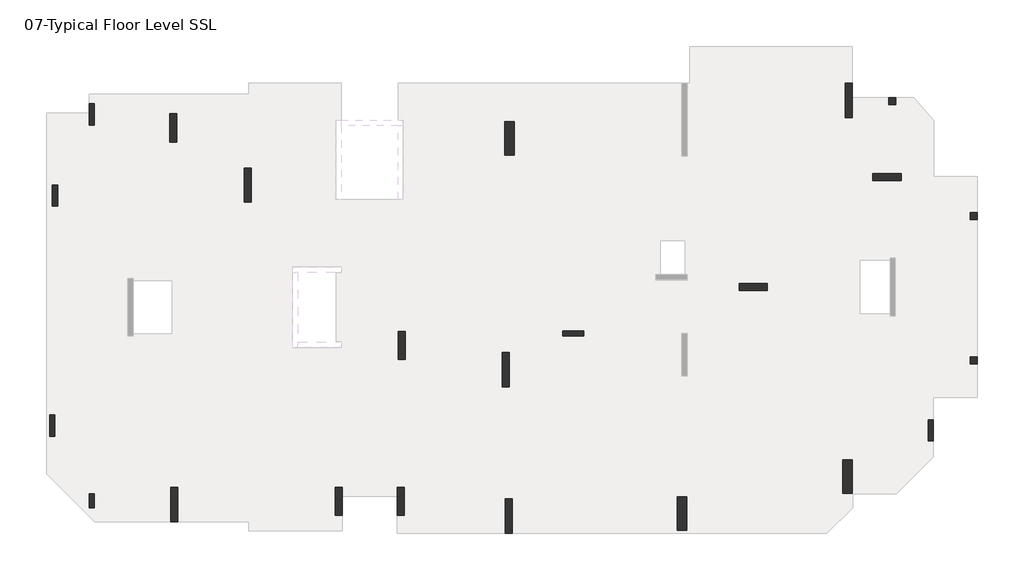
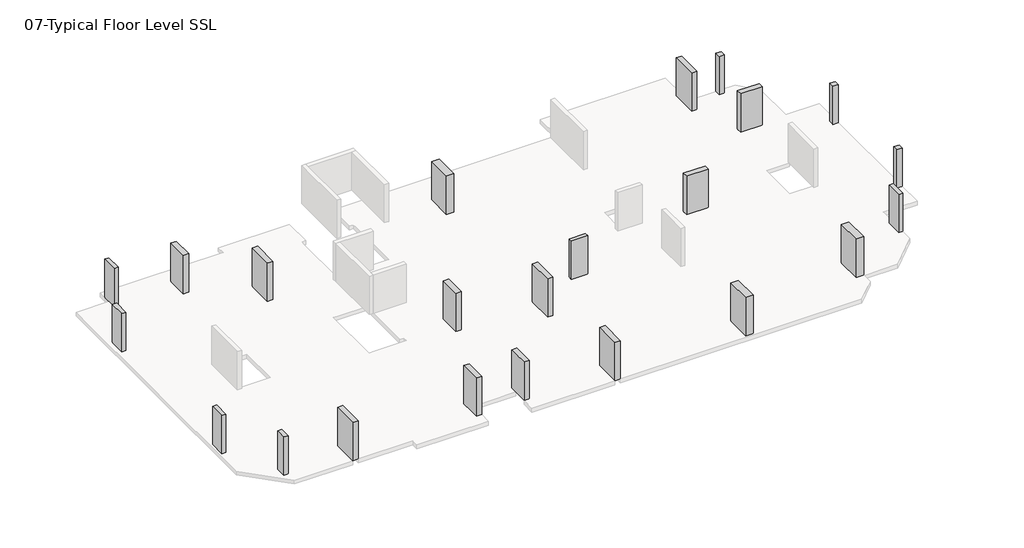
# One storey, part 2 of 2: 23 columns.
"""IFC4 building model written with IfcOpenShell, lengths in millimetres."""

from ifc_helpers import new_model, si_unit, origin, place, context, project, spatial, faceted_brep, element, save

model = new_model("IFC4")

# Units and contexts
model_context = context("Model", 3, world=origin())
ifc_project = project(units=[si_unit("LENGTHUNIT", "METRE", prefix="MILLI")], contexts=[model_context])

# Site, building, storey
site = spatial("IfcSite", under=ifc_project)
building = spatial("IfcBuilding", under=site)
storey = spatial("IfcBuildingStorey", under=building, Name="07-Typical Floor Level SSL", Elevation=15000.0)

# Columns
placement = place(None, origin())
element("IfcColumn", 1, ObjectType="M_Concrete-Rectangular-Column : C-1 (400 x 400mm)", at=placement, inside=storey, context=model_context, shape_type="Brep", body=[
    faceted_brep([(52549.9999998, 16712.0, 15000.0), (52549.9999998, 16312.0, 15000.0), (52149.9999998, 16312.0, 15000.0), (52149.9999998, 16712.0, 15000.0), (52549.9999998, 16712.0, 18000.0), (52549.9999998, 16312.0, 18000.0), (52549.9999998, 16312.0, 17700.0), (52549.9999998, 16712.0, 17700.0), (52149.9999998, 16312.0, 18000.0), (52149.9999998, 16312.0, 17700.0), (52149.9999998, 16712.0, 18000.0), (52149.9999998, 16712.0, 17700.0)], [[[0, 1, 2, 3]], [[4, 5, 6, 1, 0, 7]], [[5, 8, 9, 2, 1, 6]], [[8, 10, 11, 3, 2, 9]], [[10, 4, 7, 0, 3, 11]], [[4, 10, 8, 5]]]),
])
element("IfcColumn", 2, ObjectType="M_Concrete-Rectangular-Column : C-1 (400 x 400mm)", at=placement, inside=storey, context=model_context, shape_type="Brep", body=[
    faceted_brep([(47898.6337868, 23252.0, 15000.0), (47898.6337868, 22852.0, 15000.0), (47498.6337868, 22852.0, 15000.0), (47498.6337868, 23252.0, 15000.0), (47898.6337868, 23252.0, 18000.0), (47898.6337868, 22852.0, 18000.0), (47898.6337868, 22852.0, 17700.0), (47498.6337868, 22852.0, 18000.0), (47498.6337868, 22852.0, 17700.0), (47498.6337868, 23252.0, 18000.0)], [[[0, 1, 2, 3]], [[4, 5, 6, 1, 0]], [[5, 7, 8, 2, 1, 6]], [[7, 9, 3, 2, 8]], [[9, 4, 0, 3]], [[4, 9, 7, 5]]]),
])
element("IfcColumn", 3, ObjectType="M_Concrete-Rectangular-Column : C-1 (400 x 400mm)", at=placement, inside=storey, context=model_context, shape_type="Brep", body=[
    faceted_brep([(52549.9999998, 8504.0039609, 15000.0), (52549.9999998, 8104.0039609, 15000.0), (52149.9999998, 8104.0039609, 15000.0), (52149.9999998, 8504.0039609, 15000.0), (52549.9999998, 8504.0039609, 18000.0), (52549.9999998, 8104.0039609, 18000.0), (52549.9999998, 8104.0039609, 17700.0), (52549.9999998, 8504.0039609, 17700.0), (52149.9999998, 8104.0039609, 18000.0), (52149.9999998, 8104.0039609, 17700.0), (52149.9999998, 8504.0039609, 18000.0), (52149.9999998, 8504.0039609, 17700.0)], [[[0, 1, 2, 3]], [[4, 5, 6, 1, 0, 7]], [[5, 8, 9, 2, 1, 6]], [[8, 10, 11, 3, 2, 9]], [[10, 4, 7, 0, 3, 11]], [[4, 10, 8, 5]]]),
])
element("IfcColumn", 4, ObjectType="M_Concrete-Rectangular-Column : C-2 (300 x 800mm)", at=placement, inside=storey, context=model_context, shape_type="Brep", body=[
    faceted_brep([(2352.0, 728.0, 15000.0), (2352.0, -72.0, 15000.0), (2052.0, -72.0, 15000.0), (2052.0, 728.0, 15000.0), (2352.0, 728.0, 18000.0), (2352.0, -72.0, 18000.0), (2352.0, -72.0, 17700.0), (2352.0, 728.0, 17700.0), (2052.0, -72.0, 18000.0), (2052.0, -72.0, 17700.0), (2052.0, 728.0, 18000.0), (2052.0, 728.0, 17700.0)], [[[0, 1, 2, 3]], [[4, 5, 6, 1, 0, 7]], [[5, 8, 9, 2, 1, 6]], [[8, 10, 11, 3, 2, 9]], [[10, 4, 7, 0, 3, 11]], [[4, 10, 8, 5]]]),
])
element("IfcColumn", 5, ObjectType="M_Concrete-Rectangular-Column : C-3(300 x 1200mm)", at=placement, inside=storey, context=model_context, shape_type="Brep", body=[
    faceted_brep([(2352.0, 22908.0000656, 15000.0), (2352.0, 21708.0000656, 15000.0), (2052.0, 21708.0000656, 15000.0), (2052.0, 22908.0000656, 15000.0), (2352.0, 22908.0000656, 18000.0), (2352.0, 21708.0000656, 18000.0), (2352.0, 21708.0000656, 17700.0), (2352.0, 22908.0000656, 17700.0), (2052.0, 21708.0000656, 18000.0), (2052.0, 21708.0000656, 17700.0), (2052.0, 22380.0004589, 18000.0), (2052.0, 22908.0000656, 18000.0), (2052.0, 22908.0000656, 17700.0)], [[[0, 1, 2, 3]], [[4, 5, 6, 1, 0, 7]], [[5, 8, 9, 2, 1, 6]], [[8, 10, 11, 12, 3, 2, 9]], [[11, 4, 7, 0, 3, 12]], [[4, 11, 10, 8, 5]]]),
])
element("IfcColumn", 6, ObjectType="M_Concrete-Rectangular-Column : C-3(300 x 1200mm)", at=placement, inside=storey, context=model_context, shape_type="Brep", body=[
    faceted_brep([(257.9999999, 18288.0, 15000.0), (257.9999999, 17088.0, 15000.0), (-42.0000001, 17088.0, 15000.0), (-42.0000001, 18288.0, 15000.0), (257.9999999, 18288.0, 18000.0), (257.9999999, 17088.0, 18000.0), (257.9999999, 17088.0, 17700.0), (257.9999999, 18288.0, 17700.0), (-42.0000001, 17088.0, 18000.0), (-42.0000001, 17088.0, 17700.0), (-42.0000001, 18288.0, 18000.0), (-42.0000001, 18288.0, 17700.0)], [[[0, 1, 2, 3]], [[4, 5, 6, 1, 0, 7]], [[5, 8, 9, 2, 1, 6]], [[8, 10, 11, 3, 2, 9]], [[10, 4, 7, 0, 3, 11]], [[4, 10, 8, 5]]]),
])
element("IfcColumn", 7, ObjectType="M_Concrete-Rectangular-Column : C-3(300 x 1200mm)", at=placement, inside=storey, context=model_context, shape_type="Brep", body=[
    faceted_brep([(108.001803, 5201.9999858, 15000.0), (108.001803, 4001.9999858, 15000.0), (-191.998197, 4001.9999858, 15000.0), (-191.998197, 5201.9999858, 15000.0), (108.001803, 5201.9999858, 18000.0), (108.001803, 4001.9999858, 18000.0), (108.001803, 4001.9999858, 17700.0), (108.001803, 5201.9999858, 17700.0), (-191.998197, 4001.9999858, 18000.0), (-191.998197, 4001.9999858, 17700.0), (-191.998197, 5201.9999858, 18000.0), (-191.998197, 5201.9999858, 17700.0)], [[[0, 1, 2, 3]], [[4, 5, 6, 1, 0, 7]], [[5, 8, 9, 2, 1, 6]], [[8, 10, 11, 3, 2, 9]], [[10, 4, 7, 0, 3, 11]], [[4, 10, 8, 5]]]),
])
element("IfcColumn", 8, ObjectType="M_Concrete-Rectangular-Column : C-3(300 x 1200mm)", at=placement, inside=storey, context=model_context, shape_type="Brep", body=[
    faceted_brep([(50046.0009271, 4931.9999929, 15000.0), (50046.0009271, 3731.9999929, 15000.0), (49746.0009271, 3731.9999929, 15000.0), (49746.0009271, 4931.9999929, 15000.0), (50046.0009271, 4931.9999929, 18000.0), (50046.0009271, 3731.9999929, 18000.0), (50046.0009271, 3731.9999929, 17700.0), (50046.0009271, 4931.9999929, 17700.0), (49746.0009271, 3731.9999929, 18000.0), (49746.0009271, 3731.9999929, 17700.0), (49746.0009271, 4931.9999929, 18000.0), (49746.0009271, 4931.9999929, 17700.0)], [[[0, 1, 2, 3]], [[4, 5, 6, 1, 0, 7]], [[5, 8, 9, 2, 1, 6]], [[8, 10, 11, 3, 2, 9]], [[10, 4, 7, 0, 3, 11]], [[4, 10, 8, 5]]]),
])
element("IfcColumn", 9, ObjectType="M_Concrete-Rectangular-Column : C-3(300 x 1200mm)", at=placement, inside=storey, context=model_context, shape_type="Brep", body=[
    faceted_brep([(28975.9999998, 9996.0000019, 15000.0), (30175.9999998, 9996.0000019, 15000.0), (30175.9999998, 9696.0000019, 15000.0), (28975.9999998, 9696.0000019, 15000.0), (28975.9999998, 9996.0000019, 18000.0), (30175.9999998, 9996.0000019, 18000.0), (30175.9999998, 9996.0000019, 17700.0), (28975.9999998, 9996.0000019, 17700.0), (30175.9999998, 9696.0000019, 18000.0), (30175.9999998, 9696.0000019, 17700.0), (28975.9999998, 9696.0000019, 18000.0), (28975.9999998, 9696.0000019, 17700.0)], [[[0, 1, 2, 3]], [[4, 5, 6, 1, 0, 7]], [[5, 8, 9, 2, 1, 6]], [[8, 10, 11, 3, 2, 9]], [[10, 4, 7, 0, 3, 11]], [[4, 10, 8, 5]]]),
])
element("IfcColumn", 10, ObjectType="M_Concrete-Rectangular-Column : C-4 (400 x 1600mm)", at=placement, inside=storey, context=model_context, shape_type="Brep", body=[
    faceted_brep([(7021.9999999, 22340.0000078, 15000.0), (7021.9999999, 20740.0000078, 15000.0), (6621.9999999, 20740.0000078, 15000.0), (6621.9999999, 22340.0000078, 15000.0), (7021.9999999, 22340.0000078, 18000.0), (7021.9999999, 20740.0000078, 18000.0), (7021.9999999, 20740.0000078, 17700.0), (7021.9999999, 22340.0000078, 17700.0), (6621.9999999, 20740.0000078, 18000.0), (6621.9999999, 20740.0000078, 17700.0), (6621.9999999, 22340.0000078, 18000.0), (6621.9999999, 22340.0000078, 17700.0)], [[[0, 1, 2, 3]], [[4, 5, 6, 1, 0, 7]], [[5, 8, 9, 2, 1, 6]], [[8, 10, 11, 3, 2, 9]], [[10, 4, 7, 0, 3, 11]], [[4, 10, 8, 5]]]),
])
element("IfcColumn", 11, ObjectType="M_Concrete-Rectangular-Column : C-4 (400 x 1600mm)", at=placement, inside=storey, context=model_context, shape_type="Brep", body=[
    faceted_brep([(19969.9997488, 1087.9955348, 15000.0), (19969.9997488, -512.0044652, 15000.0), (19569.9997488, -512.0044652, 15000.0), (19569.9997488, 1087.9955348, 15000.0), (19969.9997488, 1087.9955348, 18000.0), (19969.9997488, -512.0044652, 18000.0), (19969.9997488, -512.0044652, 17700.0), (19969.9997488, 1087.9955348, 17700.0), (19569.9997488, -512.0044652, 18000.0), (19569.9997488, -512.0044652, 17700.0), (19569.9997488, 564.000519, 18000.0), (19569.9997488, 1087.9955348, 18000.0), (19569.9997488, 1087.9955348, 17700.0)], [[[0, 1, 2, 3]], [[4, 5, 6, 1, 0, 7]], [[5, 8, 9, 2, 1, 6]], [[8, 10, 11, 12, 3, 2, 9]], [[11, 4, 7, 0, 3, 12]], [[4, 11, 10, 8, 5]]]),
])
element("IfcColumn", 12, ObjectType="M_Concrete-Rectangular-Column : C-4 (400 x 1600mm)", at=placement, inside=storey, context=model_context, shape_type="Brep", body=[
    faceted_brep([(46605.9993605, 18950.0, 15000.0), (48205.9993605, 18950.0, 15000.0), (48205.9993605, 18550.0, 15000.0), (46605.9993605, 18550.0, 15000.0), (46605.9993605, 18950.0, 18000.0), (48205.9993605, 18950.0, 18000.0), (48205.9993605, 18950.0, 17700.0), (46605.9993605, 18950.0, 17700.0), (48205.9993605, 18550.0, 18000.0), (48205.9993605, 18550.0, 17700.0), (46605.9993605, 18550.0, 18000.0), (46605.9993605, 18550.0, 17700.0)], [[[0, 1, 2, 3]], [[4, 5, 6, 1, 0, 7]], [[5, 8, 9, 2, 1, 6]], [[8, 10, 11, 3, 2, 9]], [[10, 4, 7, 0, 3, 11]], [[4, 10, 8, 5]]]),
])
element("IfcColumn", 13, ObjectType="M_Concrete-Rectangular-Column : C-5 (400 x 1600mm)", at=placement, inside=storey, context=model_context, shape_type="Brep", body=[
    faceted_brep([(20030.000009, 9955.9999979, 15000.0), (20030.000009, 8355.9999979, 15000.0), (19630.000009, 8355.9999979, 15000.0), (19630.000009, 9955.9999979, 15000.0), (20030.000009, 9955.9999979, 18000.0), (20030.000009, 8355.9999979, 18000.0), (20030.000009, 8355.9999979, 17700.0), (20030.000009, 9955.9999979, 17700.0), (19630.000009, 8355.9999979, 18000.0), (19630.000009, 8355.9999979, 17700.0), (19630.000009, 9955.9999979, 18000.0), (19630.000009, 9955.9999979, 17700.0)], [[[0, 1, 2, 3]], [[4, 5, 6, 1, 0, 7]], [[5, 8, 9, 2, 1, 6]], [[8, 10, 11, 3, 2, 9]], [[10, 4, 7, 0, 3, 11]], [[4, 10, 8, 5]]]),
])
element("IfcColumn", 14, ObjectType="M_Concrete-Rectangular-Column : C-5 (400 x 1600mm)", at=placement, inside=storey, context=model_context, shape_type="Brep", body=[
    faceted_brep([(16429.9999981, 1088.0, 15000.0), (16429.9999981, -512.0, 15000.0), (16029.9999981, -512.0, 15000.0), (16029.9999981, 1088.0, 15000.0), (16429.9999981, 1088.0, 18000.0), (16429.9999981, 564.000519, 18000.0), (16429.9999981, -512.0, 18000.0), (16429.9999981, -512.0, 17700.0), (16429.9999981, 1088.0, 17700.0), (16029.9999981, -512.0, 18000.0), (16029.9999981, -512.0, 17700.0), (16029.9999981, 1088.0, 18000.0), (16029.9999981, 1088.0, 17700.0)], [[[0, 1, 2, 3]], [[4, 5, 6, 7, 1, 0, 8]], [[6, 9, 10, 2, 1, 7]], [[9, 11, 12, 3, 2, 10]], [[11, 4, 8, 0, 3, 12]], [[4, 11, 9, 6, 5]]]),
])
element("IfcColumn", 15, ObjectType="M_Concrete-Rectangular-Column : C-5 (400 x 1600mm)", at=placement, inside=storey, context=model_context, shape_type="Brep", body=[
    faceted_brep([(38998.0014887, 12692.0079212, 15000.0), (40598.0014887, 12692.0079212, 15000.0), (40598.0014887, 12292.0079212, 15000.0), (38998.0014887, 12292.0079212, 15000.0), (38998.0014887, 12692.0079212, 18000.0), (40598.0014887, 12692.0079212, 18000.0), (40598.0014887, 12692.0079212, 17700.0), (38998.0014887, 12692.0079212, 17700.0), (40598.0014887, 12292.0079212, 18000.0), (40598.0014887, 12292.0079212, 17700.0), (38998.0014887, 12292.0079212, 18000.0), (38998.0014887, 12292.0079212, 17700.0)], [[[0, 1, 2, 3]], [[4, 5, 6, 1, 0, 7]], [[5, 8, 9, 2, 1, 6]], [[8, 10, 11, 3, 2, 9]], [[10, 4, 7, 0, 3, 11]], [[4, 10, 8, 5]]]),
])
element("IfcColumn", 16, ObjectType="M_Concrete-Rectangular-Column : C-6 (400 x 1950mm)", at=placement, inside=storey, context=model_context, shape_type="Brep", body=[
    faceted_brep([(11270.0000427, 19262.9999996, 15000.0), (11270.0000427, 17312.9999996, 15000.0), (10870.0000427, 17312.9999996, 15000.0), (10870.0000427, 19262.9999996, 15000.0), (11270.0000427, 19262.9999996, 18000.0), (11270.0000427, 17312.9999996, 18000.0), (11270.0000427, 17312.9999996, 17700.0), (11270.0000427, 19262.9999996, 17700.0), (10870.0000427, 17312.9999996, 18000.0), (10870.0000427, 17312.9999996, 17700.0), (10870.0000427, 19262.9999996, 18000.0), (10870.0000427, 19262.9999996, 17700.0)], [[[0, 1, 2, 3]], [[4, 5, 6, 1, 0, 7]], [[5, 8, 9, 2, 1, 6]], [[8, 10, 11, 3, 2, 9]], [[10, 4, 7, 0, 3, 11]], [[4, 10, 8, 5]]]),
])
element("IfcColumn", 17, ObjectType="M_Concrete-Rectangular-Column : C-6 (400 x 1950mm)", at=placement, inside=storey, context=model_context, shape_type="Brep", body=[
    faceted_brep([(7082.0000416, 1083.0000153, 15000.0), (7082.0000416, -866.9999847, 15000.0), (6682.0000416, -866.9999847, 15000.0), (6682.0000416, 1083.0000153, 15000.0), (7082.0000416, 1083.0000153, 18000.0), (7082.0000416, -866.9999847, 18000.0), (7082.0000416, -866.9999847, 17700.0), (7082.0000416, 1083.0000153, 17700.0), (6682.0000416, -866.9999847, 18000.0), (6682.0000416, -866.9999847, 17700.0), (6682.0000416, 1083.0000153, 18000.0), (6682.0000416, 1083.0000153, 17700.0)], [[[0, 1, 2, 3]], [[4, 5, 6, 1, 0, 7]], [[5, 8, 9, 2, 1, 6]], [[8, 10, 11, 3, 2, 9]], [[10, 4, 7, 0, 3, 11]], [[4, 10, 8, 5]]]),
])
element("IfcColumn", 18, ObjectType="M_Concrete-Rectangular-Column : C-6 (400 x 1950mm)", at=placement, inside=storey, context=model_context, shape_type="Brep", body=[
    faceted_brep([(26113.9999998, 422.995535, 15000.0), (26113.9999998, -1527.004465, 15000.0), (25713.9999998, -1527.004465, 15000.0), (25713.9999998, 422.995535, 15000.0), (26113.9999998, 422.995535, 18000.0), (26113.9999998, -1527.004465, 18000.0), (26113.9999998, -1527.004465, 17700.0), (26113.9999998, 422.995535, 17700.0), (25713.9999998, -1527.004465, 18000.0), (25713.9999998, -1527.004465, 17700.0), (25713.9999998, 422.995535, 18000.0), (25713.9999998, 422.995535, 17700.0)], [[[0, 1, 2, 3]], [[4, 5, 6, 1, 0, 7]], [[5, 8, 9, 2, 1, 6]], [[8, 10, 11, 3, 2, 9]], [[10, 4, 7, 0, 3, 11]], [[4, 10, 8, 5]]]),
])
element("IfcColumn", 19, ObjectType="M_Concrete-Rectangular-Column : C-6 (400 x 1950mm)", at=placement, inside=storey, context=model_context, shape_type="Brep", body=[
    faceted_brep([(45446.0007483, 24087.0, 15000.0), (45446.0007483, 22137.0, 15000.0), (45046.0007483, 22137.0, 15000.0), (45046.0007483, 24087.0, 15000.0), (45446.0007483, 24087.0, 18000.0), (45446.0007483, 23252.0000315, 18000.0), (45446.0007483, 22137.0, 18000.0), (45446.0007483, 22137.0, 17700.0), (45446.0007483, 24087.0, 17700.0), (45046.0007483, 22137.0, 18000.0), (45046.0007483, 22137.0, 17700.0), (45046.0007483, 24087.0, 18000.0), (45046.0007483, 24087.0, 17700.0)], [[[0, 1, 2, 3]], [[4, 5, 6, 7, 1, 0, 8]], [[6, 9, 10, 2, 1, 7]], [[9, 11, 12, 3, 2, 10]], [[11, 4, 8, 0, 3, 12]], [[4, 11, 9, 6, 5]]]),
])
element("IfcColumn", 20, ObjectType="M_Concrete-Rectangular-Column : C-6 (400 x 1950mm)", at=placement, inside=storey, context=model_context, shape_type="Brep", body=[
    faceted_brep([(25934.0000455, 8751.0001824, 15000.0), (25934.0000455, 6801.0001824, 15000.0), (25534.0000455, 6801.0001824, 15000.0), (25534.0000455, 8751.0001824, 15000.0), (25934.0000455, 8751.0001824, 18000.0), (25934.0000455, 6801.0001824, 18000.0), (25934.0000455, 6801.0001824, 17700.0), (25934.0000455, 8751.0001824, 17700.0), (25534.0000455, 6801.0001824, 18000.0), (25534.0000455, 6801.0001824, 17700.0), (25534.0000455, 8751.0001824, 18000.0), (25534.0000455, 8751.0001824, 17700.0)], [[[0, 1, 2, 3]], [[4, 5, 6, 1, 0, 7]], [[5, 8, 9, 2, 1, 6]], [[8, 10, 11, 3, 2, 9]], [[10, 4, 7, 0, 3, 11]], [[4, 10, 8, 5]]]),
])
element("IfcColumn", 21, ObjectType="M_Concrete-Rectangular-Column : C-7 (550 x 1900mm)", at=placement, inside=storey, context=model_context, shape_type="Brep", body=[
    faceted_brep([(36035.9999998, 548.0007983, 15000.0), (36035.9999998, -1351.9992017, 15000.0), (35485.9999998, -1351.9992017, 15000.0), (35485.9999998, 548.0007983, 15000.0), (36035.9999998, 548.0007983, 18000.0), (36035.9999998, -1351.9992017, 18000.0), (36035.9999998, -1351.9992017, 17700.0), (36035.9999998, 548.0007983, 17700.0), (35485.9999998, -1351.9992017, 18000.0), (35485.9999998, -1351.9992017, 17700.0), (35485.9999998, 548.0007983, 18000.0), (35485.9999998, 548.0007983, 17700.0)], [[[0, 1, 2, 3]], [[4, 5, 6, 1, 0, 7]], [[5, 8, 9, 2, 1, 6]], [[8, 10, 11, 3, 2, 9]], [[10, 4, 7, 0, 3, 11]], [[4, 10, 8, 5]]]),
])
element("IfcColumn", 22, ObjectType="M_Concrete-Rectangular-Column : C-7 (550 x 1900mm)", at=placement, inside=storey, context=model_context, shape_type="Brep", body=[
    faceted_brep([(45443.9999998, 2648.0, 15000.0), (45443.9999998, 748.0, 15000.0), (44893.9999998, 748.0, 15000.0), (44893.9999998, 2648.0, 15000.0), (45443.9999998, 2648.0, 18000.0), (45443.9999998, 748.0, 18000.0), (45443.9999998, 748.0, 17700.0), (45443.9999998, 2648.0, 17700.0), (44893.9999998, 748.0, 18000.0), (44893.9999998, 748.0, 17700.0), (44893.9999998, 2648.0, 18000.0), (44893.9999998, 2648.0, 17700.0)], [[[0, 1, 2, 3]], [[4, 5, 6, 1, 0, 7]], [[5, 8, 9, 2, 1, 6]], [[8, 10, 11, 3, 2, 9]], [[10, 4, 7, 0, 3, 11]], [[4, 10, 8, 5]]]),
])
element("IfcColumn", 23, ObjectType="M_Concrete-Rectangular-Column : C-7 (550 x 1900mm)", at=placement, inside=storey, context=model_context, shape_type="Brep", body=[
    faceted_brep([(26218.9999998, 21900.0, 15000.0), (26218.9999998, 20000.0, 15000.0), (25668.9999998, 20000.0, 15000.0), (25668.9999998, 21900.0, 15000.0), (26218.9999998, 21900.0, 18000.0), (26218.9999998, 20000.0, 18000.0), (26218.9999998, 20000.0, 17700.0), (26218.9999998, 21900.0, 17700.0), (25668.9999998, 20000.0, 18000.0), (25668.9999998, 20000.0, 17700.0), (25668.9999998, 21900.0, 18000.0), (25668.9999998, 21900.0, 17700.0)], [[[0, 1, 2, 3]], [[4, 5, 6, 1, 0, 7]], [[5, 8, 9, 2, 1, 6]], [[8, 10, 11, 3, 2, 9]], [[10, 4, 7, 0, 3, 11]], [[4, 10, 8, 5]]]),
])

save(model, "model.ifc")

# Revit data of these elements
# Type "M_Concrete-Rectangular-Column : C-1 (400 x 400mm)"
#   Type Mark = "C01"
#   b = 400 mm
#   h = 400 mm
#   Structural Material [instance default] = Concrete, Cast-in-Place gray
# Type "M_Concrete-Rectangular-Column : C-2 (300 x 800mm)"
#   Type Mark = "C02"
#   b = 300 mm
#   h = 800 mm
#   Structural Material [instance default] = Concrete, Cast-in-Place gray
# Type "M_Concrete-Rectangular-Column : C-3(300 x 1200mm)"
#   Type Mark = "C03"
#   b = 300 mm
#   h = 1200 mm
#   Structural Material [instance default] = Concrete, Cast-in-Place gray
# Type "M_Concrete-Rectangular-Column : C-4 (400 x 1600mm)"
#   Type Mark = "C04"
#   b = 400 mm
#   h = 1600 mm
#   Structural Material [instance default] = Concrete, Cast-in-Place gray
# Type "M_Concrete-Rectangular-Column : C-5 (400 x 1600mm)"
#   Type Mark = "C05"
#   b = 400 mm
#   h = 1600 mm
#   Structural Material [instance default] = Concrete, Cast-in-Place gray
# Type "M_Concrete-Rectangular-Column : C-6 (400 x 1950mm)"
#   Type Mark = "C06"
#   b = 400 mm
#   h = 1950 mm
#   Structural Material [instance default] = Concrete, Cast-in-Place gray
# Type "M_Concrete-Rectangular-Column : C-7 (550 x 1900mm)"
#   Type Mark = "C07"
#   b = 550 mm
#   h = 1900 mm
#   Structural Material [instance default] = Concrete, Cast-in-Place gray
# Elements 1, 2, 3 (IfcColumn, "M_Concrete-Rectangular-Column : C-1 (400 x 400mm)")
#   Structural Material = Concrete-RC
#   Phase Created = New Construction
#   Materials on its faces: "Concrete-RC"
# Element 4 (IfcColumn, "M_Concrete-Rectangular-Column : C-2 (300 x 800mm)")
#   Structural Material = Concrete-RC
#   Phase Created = New Construction
#   Materials on its faces: "Concrete-RC"
# Elements 5, 6, 7, 8, 9 (IfcColumn, "M_Concrete-Rectangular-Column : C-3(300 x 1200mm)")
#   Structural Material = Concrete-RC
#   Phase Created = New Construction
#   Materials on its faces: "Concrete-RC"
# Elements 10, 11, 12 (IfcColumn, "M_Concrete-Rectangular-Column : C-4 (400 x 1600mm)")
#   Structural Material = Concrete-RC
#   Phase Created = New Construction
#   Materials on its faces: "Concrete-RC"
# Elements 13, 14, 15 (IfcColumn, "M_Concrete-Rectangular-Column : C-5 (400 x 1600mm)")
#   Structural Material = Concrete-RC
#   Phase Created = New Construction
#   Materials on its faces: "Concrete-RC"
# Elements 16, 17, 18, 19, 20 (IfcColumn, "M_Concrete-Rectangular-Column : C-6 (400 x 1950mm)")
#   Structural Material = Concrete-RC
#   Phase Created = New Construction
#   Materials on its faces: "Concrete-RC"
# Elements 21, 22, 23 (IfcColumn, "M_Concrete-Rectangular-Column : C-7 (550 x 1900mm)")
#   Structural Material = Concrete-RC
#   Phase Created = New Construction
#   Materials on its faces: "Concrete-RC"
# Materials
#   "Concrete, Cast-in-Place gray": class "Concrete", colour RGB 192 192 192, transparency 0, Description = "Cast-in-place concrete", Cost = 0
#   "Concrete-RC": class "Concrete", colour RGB 128 128 128, transparency 0, Description = "High strength concrete", Cost = 0
